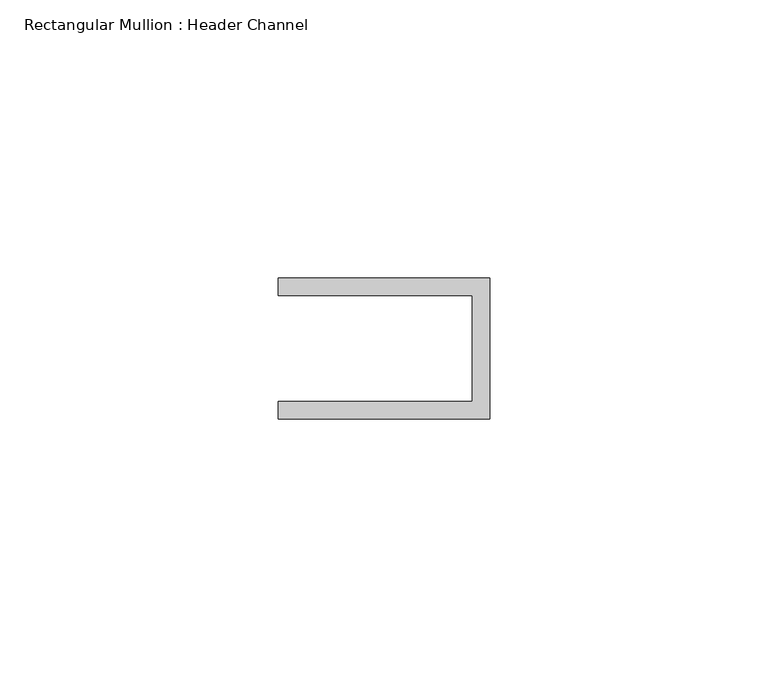
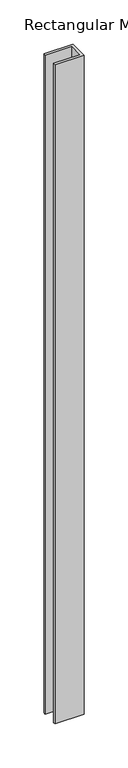
"""IFC4 building model written with IfcOpenShell, lengths in millimetres: member geometry, Rectangular Mullion : Header Channel."""

import ifcopenshell
import ifcopenshell.guid

model = None  # the IFC model being written
_history = None  # IfcOwnerHistory: only IFC2X3 demands one
_inside = {}  # id of a spatial element -> (the spatial element, [elements in it])
_under = {}  # id of a project, library or spatial element -> (it, [spatial elements below it])
_declared = {}  # id of a project -> (the project, [libraries it declares])
_typed = {}  # id of a type object -> (the type object, [elements of that type])
_made_of = {}  # id of a material, layer set ... -> (it, [elements and type objects made of it])


def new_model(schema):
    """Start an empty IFC model of exactly this schema.

    Asked for "IFC4X3", IfcOpenShell would pick the latest addendum, in which some entities
    have other attributes; the version numbers below select the first issue.
    IFC2X3 requires an IfcOwnerHistory on every rooted entity: one is made here for all.
    """
    global model, _history
    if schema == "IFC4X3":
        model = ifcopenshell.file(schema_version=(4, 3, 0, 0))
    else:
        model = ifcopenshell.file(schema=schema)
    _inside.clear()
    _under.clear()
    _declared.clear()
    _typed.clear()
    _made_of.clear()
    _history = None
    if model.schema == "IFC2X3":
        org = make("IfcOrganization", Name="unknown")
        user = make(
            "IfcPersonAndOrganization",
            ThePerson=make("IfcPerson", FamilyName="unknown"),
            TheOrganization=org,
        )
        app = make(
            "IfcApplication",
            ApplicationDeveloper=org,
            Version="unknown",
            ApplicationFullName="unknown",
            ApplicationIdentifier="unknown",
        )
        _history = make(
            "IfcOwnerHistory",
            OwningUser=user,
            OwningApplication=app,
            ChangeAction="ADDED",
            CreationDate=0,
        )
    return model


def make(cls, **values):
    """One entity of the class cls with the attributes given. An attribute that is None is left unset."""
    return model.create_entity(
        cls, **{name: value for name, value in values.items() if value is not None}
    )


def rooted(cls, **values):
    """An entity with a GlobalId (a new one), such as an element, a storey or a relation."""
    return make(cls, GlobalId=ifcopenshell.guid.new(), OwnerHistory=_history, **values)


def si_unit(unit_type, name, prefix=None):
    """IfcSIUnit, for example si_unit("LENGTHUNIT", "METRE", prefix="MILLI")."""
    return make("IfcSIUnit", UnitType=unit_type, Prefix=prefix, Name=name)


def assignment(units):
    """IfcUnitAssignment: the units of a project."""
    return None if units is None else make("IfcUnitAssignment", Units=units)


def point(xyz):
    """IfcCartesianPoint."""
    return None if xyz is None else make("IfcCartesianPoint", Coordinates=xyz)


def direction(xyz):
    """IfcDirection."""
    return None if xyz is None else make("IfcDirection", DirectionRatios=xyz)


def frame(location, z_axis=None, x_axis=None):
    """IfcAxis2Placement3D, a coordinate frame: its origin and axes. An axis left out is left unset."""
    return make(
        "IfcAxis2Placement3D",
        Location=point(location),
        Axis=direction(z_axis),
        RefDirection=direction(x_axis),
    )


def origin():
    """The frame at (0, 0, 0) with its axes left unset."""
    return frame((0.0, 0.0, 0.0))


def place(relative_to, where):
    """IfcLocalPlacement: puts the frame where relative to a parent placement (None: the world)."""
    return make(
        "IfcLocalPlacement", PlacementRelTo=relative_to, RelativePlacement=where
    )


def context(
    kind, dimensions, precision=None, world=None, true_north=None, identifier=None
):
    """IfcGeometricRepresentationContext, for example the 3D "Model" context."""
    return make(
        "IfcGeometricRepresentationContext",
        ContextIdentifier=identifier,
        ContextType=kind,
        CoordinateSpaceDimension=dimensions,
        Precision=precision,
        WorldCoordinateSystem=world,
        TrueNorth=true_north,
    )


def project(units=None, contexts=None):
    """IfcProject with its units and contexts."""
    return rooted(
        "IfcProject",
        Name="project",
        RepresentationContexts=contexts,
        UnitsInContext=assignment(units),
    )


def spatial(cls, under=None, at=None, **own):
    """A site, building, storey or space (cls), placed at a placement, below another one or the project."""
    s = rooted(cls, ObjectPlacement=at, **own)
    if under is not None:
        _under.setdefault(under.id(), (under, []))[1].append(s)
    return s


def polyline(points):
    """IfcPolyline through the points."""
    return make("IfcPolyline", Points=[point(p) for p in points])


def outline(outer, holes=None, kind="AREA"):
    """IfcArbitraryClosedProfileDef: a profile drawn as a closed curve; with holes, ...WithVoids."""
    if holes is None:
        return make("IfcArbitraryClosedProfileDef", ProfileType=kind, OuterCurve=outer)
    return make(
        "IfcArbitraryProfileDefWithVoids",
        ProfileType=kind,
        OuterCurve=outer,
        InnerCurves=holes,
    )


def extrude(swept, where, along, depth):
    """IfcExtrudedAreaSolid: the profile swept, set in the frame where, extruded along a direction by depth."""
    return make(
        "IfcExtrudedAreaSolid",
        SweptArea=swept,
        Position=where,
        ExtrudedDirection=direction(along),
        Depth=depth,
    )


def shape(context_of_items, identifier, shape_type, items):
    """IfcShapeRepresentation: the items that make up one representation, for example the "Body"."""
    return make(
        "IfcShapeRepresentation",
        ContextOfItems=context_of_items,
        RepresentationIdentifier=identifier,
        RepresentationType=shape_type,
        Items=items,
    )


def source(mapping_origin, context_of_items, identifier, shape_type, items):
    """IfcRepresentationMap: a shape defined once, which mapped items show again and again."""
    return make(
        "IfcRepresentationMap",
        MappingOrigin=mapping_origin,
        MappedRepresentation=shape(context_of_items, identifier, shape_type, items),
    )


def transform(
    local_origin,
    x_axis=None,
    y_axis=None,
    z_axis=None,
    scale=None,
    scale2=None,
    scale3=None,
    uniform=True,
):
    """IfcCartesianTransformationOperator3D, or its non-uniform kind. x_axis, y_axis, z_axis: its Axis1, 2, 3."""
    if uniform:
        return make(
            "IfcCartesianTransformationOperator3D",
            Axis1=direction(x_axis),
            Axis2=direction(y_axis),
            LocalOrigin=point(local_origin),
            Scale=scale,
            Axis3=direction(z_axis),
        )
    return make(
        "IfcCartesianTransformationOperator3DnonUniform",
        Axis1=direction(x_axis),
        Axis2=direction(y_axis),
        LocalOrigin=point(local_origin),
        Scale=scale,
        Axis3=direction(z_axis),
        Scale2=scale2,
        Scale3=scale3,
    )


def mapped(mapping_source, mapping_target):
    """IfcMappedItem: shows the shape of a source again, moved by a transform."""
    return make(
        "IfcMappedItem", MappingSource=mapping_source, MappingTarget=mapping_target
    )


def made_of(thing, what):
    """Note that an element or type object is made of a material, layer set ...; save() writes the relation."""
    if what is not None:
        _made_of.setdefault(what.id(), (what, []))[1].append(thing)
    return thing


def element(
    cls,
    number,
    at=None,
    inside=None,
    cuts=None,
    type_object=None,
    material=None,
    context=None,
    identifier="Body",
    shape_type=None,
    held_by="IfcProductDefinitionShape",
    body=None,
    shapes=None,
    **own,
):
    """One element of the class cls, such as IfcWall. Its Tag is "e" and its number.

    at: its placement. inside: the storey or other place that contains it. cuts: it is an
    opening in that element (IfcRelVoidsElement). A single representation is given by context,
    identifier, shape_type and body (its items); several are given by shapes. held_by: the class
    of the entity that holds the representations. save() writes the other relations.
    """
    e = rooted(cls, Tag="e%d" % number, ObjectPlacement=at, **own)
    if body is not None:
        shapes = [shape(context, identifier, shape_type, body)]
    if shapes is not None:
        e.Representation = make(held_by, Representations=shapes)
    if inside is not None:
        _inside.setdefault(inside.id(), (inside, []))[1].append(e)
    if cuts is not None:
        rooted(
            "IfcRelVoidsElement", RelatingBuildingElement=cuts, RelatedOpeningElement=e
        )
    if type_object is not None:
        _typed.setdefault(type_object.id(), (type_object, []))[1].append(e)
    return made_of(e, material)


def aggregate(whole, parts):
    """IfcRelAggregates: a whole, such as a stair, and the parts it consists of."""
    return rooted("IfcRelAggregates", RelatingObject=whole, RelatedObjects=parts)


def save(model, path):
    """Write the relations noted so far, then the file.

    IfcRelAggregates (storeys below a building ...), IfcRelContainedInSpatialStructure (elements
    in a storey), IfcRelDefinesByType, IfcRelAssociatesMaterial and IfcRelDeclares: one each for
    every whole, place, type object, material and project.
    """
    for whole, parts in _under.values():
        aggregate(whole, parts)
    for where, things in _inside.values():
        rooted(
            "IfcRelContainedInSpatialStructure",
            RelatedElements=things,
            RelatingStructure=where,
        )
    for kind, things in _typed.values():
        rooted("IfcRelDefinesByType", RelatedObjects=things, RelatingType=kind)
    for what, things in _made_of.values():
        rooted("IfcRelAssociatesMaterial", RelatedObjects=things, RelatingMaterial=what)
    for by, libraries in _declared.values():
        rooted("IfcRelDeclares", RelatingContext=by, RelatedDefinitions=libraries)
    model.write(path)


def rectangular_mullion_header_channel_4f4c83a4(model_context):
    return source(origin(), model_context, "Body", "SweptSolid", [
        extrude(outline(polyline([(0.0, -12.7), (-38.1, -12.7), (-38.1, -9.525), (-3.175, -9.525), (-3.175, 9.525), (-38.1, 9.525), (-38.1, 12.7), (0.0, 12.7), (0.0, -12.7)])), frame((0.0, 0.0, -914.4), z_axis=(0.0, 0.0, 1.0), x_axis=(1.0, 0.0, 0.0)), (0.0, 0.0, 1.0), 914.4),
    ])


if __name__ == "__main__":
    model = new_model("IFC4")
    model_context = context("Model", 3, world=origin())
    ifc_project = project(units=[si_unit("LENGTHUNIT", "METRE", prefix="MILLI")], contexts=[model_context])
    site = spatial("IfcSite", under=ifc_project)
    building = spatial("IfcBuilding", under=site)
    placement = place(None, origin())
    rectangular_mullion_header_channel_shape = rectangular_mullion_header_channel_4f4c83a4(model_context)
    element("IfcMember", 1, ObjectType="Rectangular Mullion : Header Channel", at=placement, inside=building, context=model_context, shape_type="MappedRepresentation", body=[
        mapped(rectangular_mullion_header_channel_shape, transform((0.0, 0.0, 0.0), x_axis=(1.0, 0.0, 0.0), y_axis=(0.0, 1.0, 0.0), z_axis=(0.0, 0.0, 1.0))),
    ])
    save(model, "model.ifc")

# Revit data of these elements
# Type "Rectangular Mullion : Header Channel"
#   built-in parameter 1007322 = 0.0833333 (stored number, unit not read)
#   built-in parameter 1007321 = -0.03125 (stored number, unit not read)
#   built-in parameter 1007320 = 0.0416667 (stored number, unit not read)
# Element 1 (IfcMember, "Rectangular Mullion : Header Channel")
#   Materials on its faces: "ALUM"
# Materials
#   "ALUM": class "Generic", colour RGB 157 157 157, transparency 0, Cost = 0
